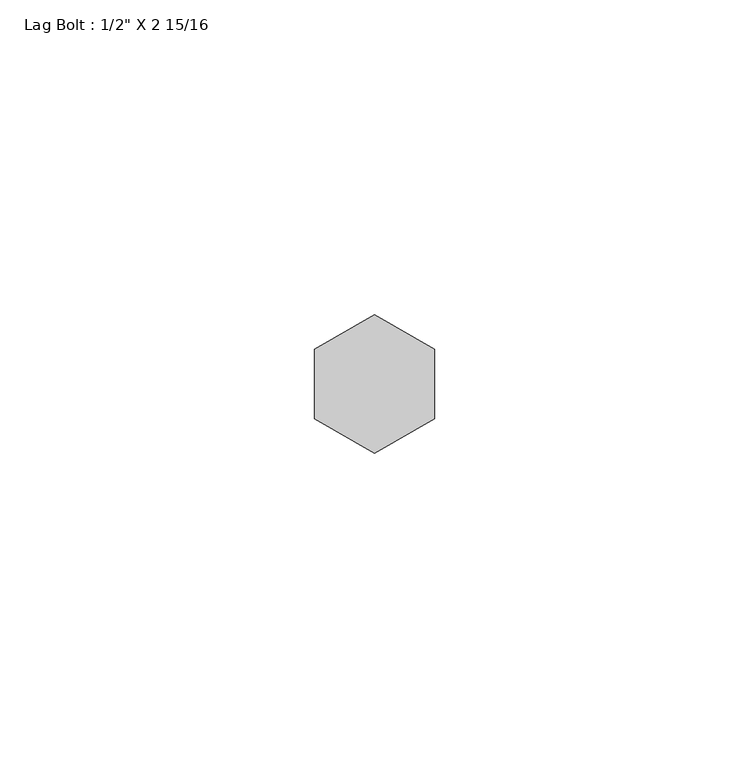
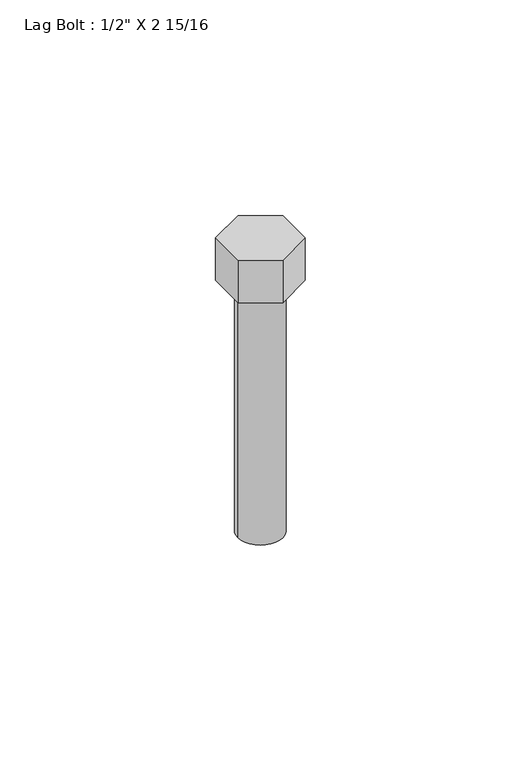
"""IFC4 building model written with IfcOpenShell, lengths in millimetres: proxy geometry."""

from ifc_helpers import new_model, si_unit, point, frame, origin, origin_with_axes, origin_2d, place, context, project, spatial, polyline, circle_curve, trimmed, segment, composite_curve, outline, extrude, source, transform, mapped, element, save


def proxy_10e277fe(model_context):
    return source(origin(), model_context, "Body", "SweptSolid", [
        extrude(outline(polyline([(-9.525, 5.4992613), (0.0, 10.9985226), (9.525, 5.4992613), (9.525, -5.4992613), (0.0, -10.9985226), (-9.525, -5.4992613), (-9.525, 5.4992613)])), origin_with_axes(), (0.0, 0.0, 1.0), 12.7),
        extrude(outline(composite_curve([segment(trimmed(circle_curve(origin_2d(), 6.35), [point((-6.35, 0.0))], [point((6.35, 0.0))], False, "CARTESIAN"), True, "CONTINUOUS"), segment(trimmed(circle_curve(origin_2d(), 6.35), [point((6.35, 0.0))], [point((-6.35, 0.0))], False, "CARTESIAN"), True, "CONTINUOUS")], self_intersect=False)), frame((0.0, 0.0, -74.6125), z_axis=(0.0, 0.0, 1.0), x_axis=(1.0, 0.0, 0.0)), (0.0, 0.0, 1.0), 74.6125),
    ])


if __name__ == "__main__":
    model = new_model("IFC4")
    model_context = context("Model", 3, world=origin())
    ifc_project = project(units=[si_unit("LENGTHUNIT", "METRE", prefix="MILLI")], contexts=[model_context])
    site = spatial("IfcSite", under=ifc_project)
    building = spatial("IfcBuilding", under=site)
    placement = place(None, origin())
    proxy_shape = proxy_10e277fe(model_context)
    element("IfcBuildingElementProxy", 1, Name="Lag Bolt : 1/2\" X 2 15/16", ObjectType="Lag Bolt : 1/2\" X 2 15/16", at=placement, inside=building, context=model_context, shape_type="MappedRepresentation", body=[
        mapped(proxy_shape, transform((0.0, 0.0, 0.0), x_axis=(1.0, 0.0, 0.0), y_axis=(0.0, 1.0, 0.0), z_axis=(0.0, 0.0, 1.0))),
    ])
    save(model, "model.ifc")

# Revit data of these elements
# Type "Lag Bolt : 1/2\" X 2 15/16"
#   Thickness_of_Substrate [instance default] = 0' - 1"
#   Side = 0' - 0 111/256"
#   Radius = 0' - 0 1/4"
#   Length = 0' - 2 15/16"
#   Head Size = 0' - 0 3/4"
#   Head Radius = 0' - 0 3/8"
#   Head Height = 0' - 0 1/2"
#   Diameter = 0' - 0 1/2"
#   Default Elevation = 4' - 0"
#   Nut_Visibility [instance default] = yes
#   Bolt Material (Size) [instance default] = 1/2" X 5" LAG BOLT (THRU BOLT IF PLATE ON OPP. SIDE OF STRUCT MEMBER)
# Element 1 (IfcBuildingElementProxy, "Lag Bolt : 1/2\" X 2 15/16")
#   Nut_Visibility = no
#   Bolt Material (Size) = THRU-BOLT OR LAG BOLT
#   Materials on its faces: "THRU-BOLT OR LAG BOLT"
# Materials
#   "1/2\" X 5\" LAG BOLT (THRU BOLT IF PLATE ON OPP. SIDE OF STRUCT MEMBER)": class "Generic", colour RGB 120 120 120, transparency 0, Cost = 0
#   "THRU-BOLT OR LAG BOLT": class "Generic", colour RGB 120 120 120, transparency 0, Cost = 0
